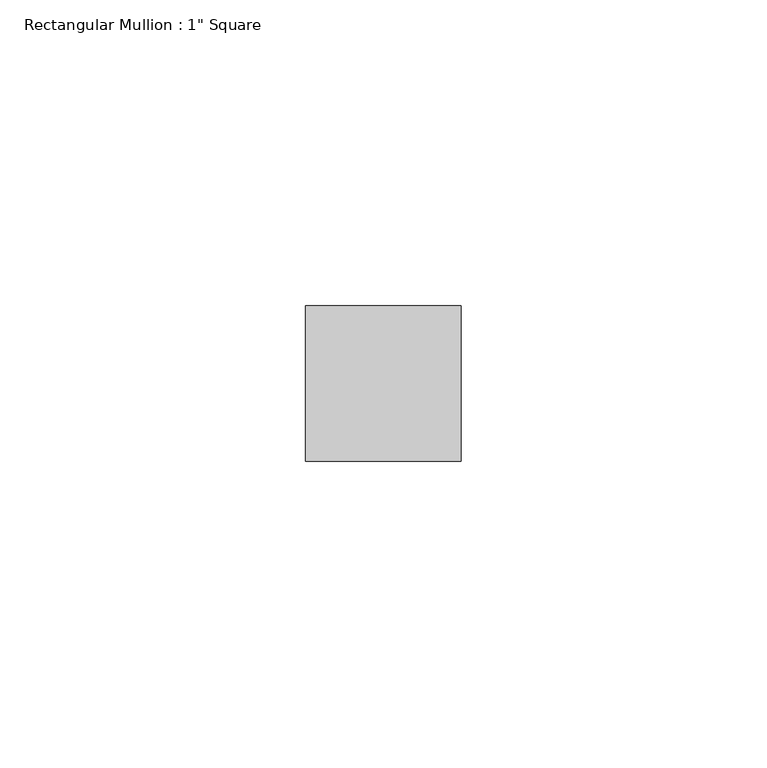
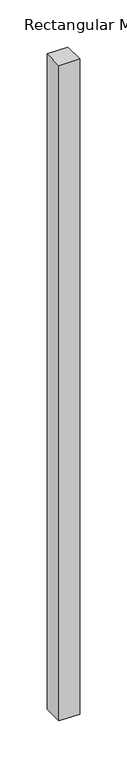
"""IFC4 building model written with IfcOpenShell, lengths in millimetres: member geometry."""

from ifc_helpers import new_model, si_unit, frame, origin, place, context, project, spatial, polyline, outline, extrude, source, transform, mapped, element, save


def member_7b999d6d(model_context):
    return source(origin(), model_context, "Body", "SweptSolid", [
        extrude(outline(polyline([(12.7, 12.7), (12.7, -12.7), (-12.7, -12.7), (-12.7, 12.7), (12.7, 12.7)])), frame((0.0, 0.0, -850.8999997), z_axis=(0.0, 0.0, 1.0), x_axis=(1.0, 0.0, 0.0)), (0.0, 0.0, 1.0), 850.8999997),
    ])


if __name__ == "__main__":
    model = new_model("IFC4")
    model_context = context("Model", 3, world=origin())
    ifc_project = project(units=[si_unit("LENGTHUNIT", "METRE", prefix="MILLI")], contexts=[model_context])
    site = spatial("IfcSite", under=ifc_project)
    building = spatial("IfcBuilding", under=site)
    placement = place(None, origin())
    member_shape = member_7b999d6d(model_context)
    element("IfcMember", 1, ObjectType="Rectangular Mullion : 1\" Square", at=placement, inside=building, context=model_context, shape_type="MappedRepresentation", body=[
        mapped(member_shape, transform((0.0, 0.0, 0.0), x_axis=(1.0, 0.0, 0.0), y_axis=(0.0, 1.0, 0.0), z_axis=(0.0, 0.0, 1.0))),
    ])
    save(model, "model.ifc")

# Revit data of these elements
# Type "Rectangular Mullion : 1\" Square"
#   built-in parameter 1007304 = 0.0833333 (stored number, unit not read)
#   built-in parameter 1007301 = 0.0416667 (stored number, unit not read)
#   built-in parameter 1007300 = 0.0416667 (stored number, unit not read)
# Element 1 (IfcMember, "Rectangular Mullion : 1\" Square")
#   Materials on its faces: "Metal - Aluminum"
# Materials
#   "Metal - Aluminum": class "Metal", colour RGB 247 247 247, transparency 0
